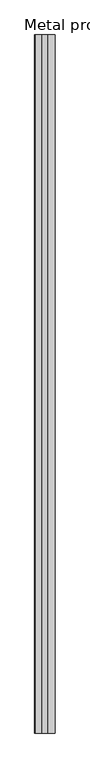
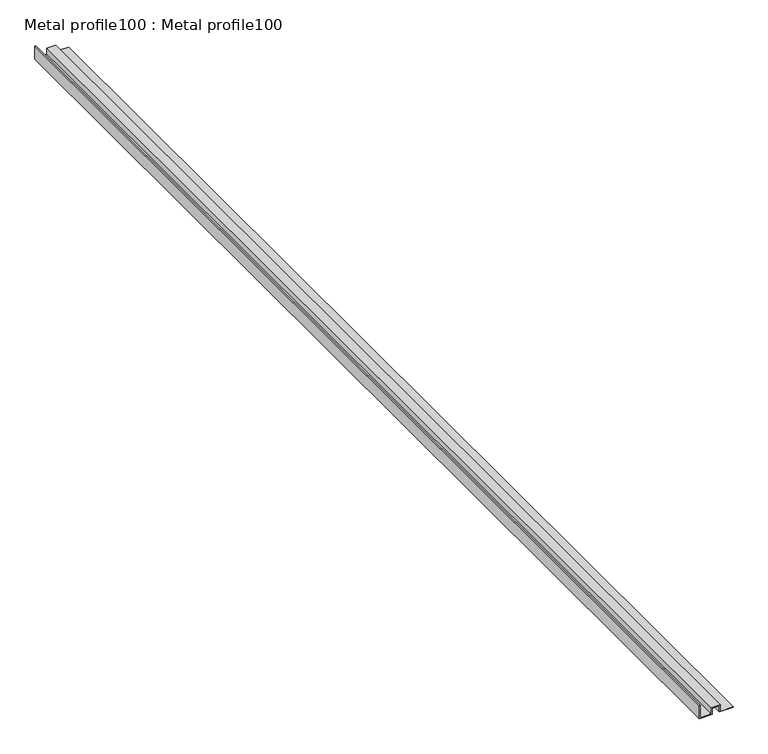
"""IFC4 building model written with IfcOpenShell, lengths in millimetres: proxy geometry, Metal profile100 : Metal profile100."""

from ifc_helpers import new_model, si_unit, frame, origin, place, context, project, spatial, polyline, outline, extrude, source, transform, mapped, element, save


def metal_profile100_metal_profile100_949488a8(model_context):
    return source(origin(), model_context, "Body", "SweptSolid", [
        extrude(outline(polyline([(35054.4375625, -8454.9125717), (35054.4375625, -8432.6875717), (35065.8675625, -8432.6875717), (35065.8675625, -8419.9875717), (35054.4375625, -8419.9875717), (35054.4375625, -8396.2743878), (35055.7175625, -8396.2743878), (35055.7175625, -8418.7075717), (35067.1475625, -8418.7075717), (35067.1475625, -8433.9675717), (35055.7175625, -8433.9675717), (35055.7175625, -8453.6325717), (35078.238324, -8453.6325717), (35078.238324, -8454.9125717), (35054.4375625, -8454.9125717)])), frame((0.0, 4540.4513244, 0.0), z_axis=(0.0, 1.0, 0.0), x_axis=(0.0, 0.0, 1.0)), (0.0, 0.0, 1.0), 2000.0),
    ])


if __name__ == "__main__":
    model = new_model("IFC4")
    model_context = context("Model", 3, world=origin())
    ifc_project = project(units=[si_unit("LENGTHUNIT", "METRE", prefix="MILLI")], contexts=[model_context])
    site = spatial("IfcSite", under=ifc_project)
    building = spatial("IfcBuilding", under=site)
    placement = place(None, origin())
    metal_profile100_metal_profile100_shape = metal_profile100_metal_profile100_949488a8(model_context)
    element("IfcBuildingElementProxy", 1, Name="Metal profile100 : Metal profile100", ObjectType="Metal profile100 : Metal profile100", at=placement, inside=building, context=model_context, shape_type="MappedRepresentation", body=[
        mapped(metal_profile100_metal_profile100_shape, transform((0.0, 0.0, 0.0), x_axis=(1.0, 0.0, 0.0), y_axis=(0.0, 1.0, 0.0), z_axis=(0.0, 0.0, 1.0))),
    ])
    save(model, "model.ifc")

# Revit data of these elements
# Type "Metal profile100 : Metal profile100"
#   NameOverride = "Metal profile100"
# Element 1 (IfcBuildingElementProxy, "Metal profile100 : Metal profile100")
#   Materials on its faces: "16 GA. COPPER SOFFIT DRIP SCREED"
# Materials
#   "16 GA. COPPER SOFFIT DRIP SCREED": class "Unassigned", colour RGB 255 217 0, transparency 0
